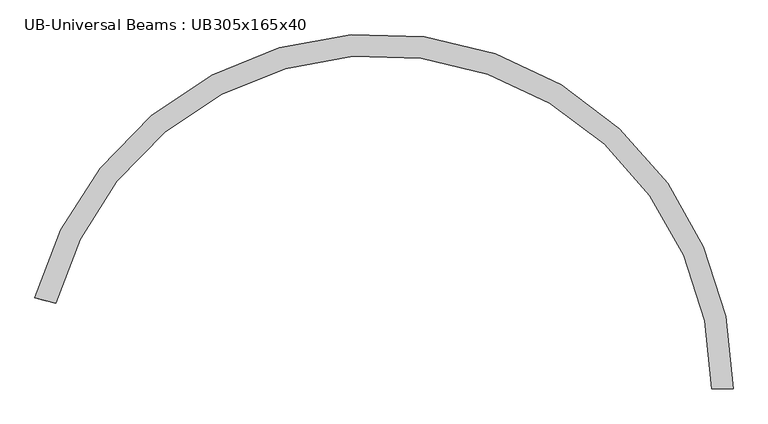
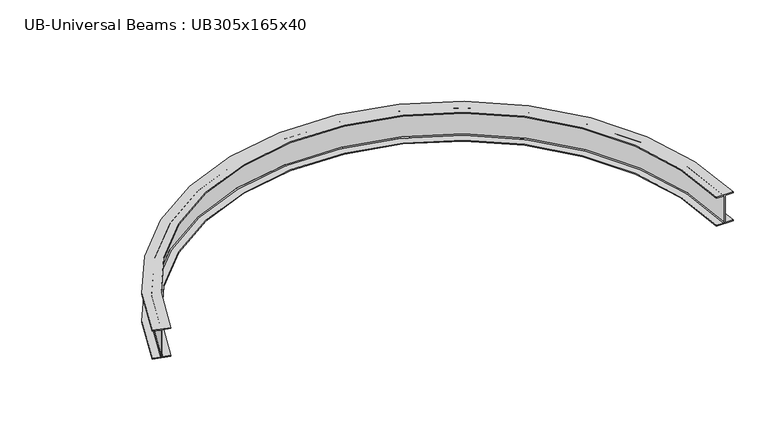
"""IFC4 building model written with IfcOpenShell, lengths in millimetres: beam geometry, UB-Universal Beams : UB305x165x40."""

from ifc_helpers import new_model, si_unit, point, frame, origin, place, context, project, spatial, polyline, circle_curve, ellipse_curve, trimmed, source, transform, mapped, element, save
from ifc_brep_helpers import plane_surface, cylinder_surface, revolved_surface, advanced_brep


def ub_universal_beams_ub305x165x40_4e4f8f72(model_context):
    return source(origin(), model_context, "Body", "AdvancedBrep", [
        advanced_brep(
        [(2724.4689627, -2641.9689627, -141.5), (2653.8689627, -2641.9689627, -141.5), (2644.9689627, -2641.9689627, -132.6), (2644.9689627, -2641.9689627, 132.6), (2653.8689627, -2641.9689627, 141.5), (2724.4689627, -2641.9689627, 141.5), (2724.4689627, -2641.9689627, 151.7), (2559.4689627, -2641.9689627, 151.7), (2559.4689627, -2641.9689627, 141.5), (2630.0689627, -2641.9689627, 141.5), (2638.9689627, -2641.9689627, 132.6), (2638.9689627, -2641.9689627, -132.6), (2630.0689627, -2641.9689627, -141.5), (2559.4689627, -2641.9689627, -141.5), (2559.4689627, -2641.9689627, -151.7), (2724.4689627, -2641.9689627, -151.7), (-2633.0924312, -1942.2866222, -141.5), (-2633.0924312, -1942.2866222, -151.7), (-2473.6264005, -1984.6609666, -151.7), (-2473.6264005, -1984.6609666, -141.5), (-2541.8585324, -1966.5298835, -141.5), (-2550.4600335, -1964.244237, -132.6), (-2550.4600335, -1964.244237, 132.6), (-2541.8585324, -1966.5298835, 141.5), (-2473.6264005, -1984.6609666, 141.5), (-2473.6264005, -1984.6609666, 151.7), (-2633.0924312, -1942.2866222, 151.7), (-2633.0924312, -1942.2866222, 141.5), (-2564.8602993, -1960.4177053, 141.5), (-2556.2587982, -1962.7033518, 132.6), (-2556.2587982, -1962.7033518, -132.6), (-2564.8602993, -1960.4177053, -141.5)],
        [
            (0, 1),
            (1, 2, circle_curve(frame((2653.8689627, -2641.9689627, -132.6), z_axis=(0.0, 1.0, 0.0), x_axis=(-1.0, 0.0, 0.0)), 8.9)),
            (2, 3),
            (3, 4, circle_curve(frame((2653.8689627, -2641.9689627, 132.6), z_axis=(0.0, 1.0, 0.0), x_axis=(-1.0, 0.0, 0.0)), 8.9)),
            (4, 5),
            (5, 6),
            (6, 7),
            (7, 8),
            (8, 9),
            (9, 10, circle_curve(frame((2630.0689627, -2641.9689627, 132.6), z_axis=(0.0, 1.0, 0.0), x_axis=(-1.0, 0.0, 0.0)), 8.9)),
            (10, 11),
            (11, 12, circle_curve(frame((2630.0689627, -2641.9689627, -132.6), z_axis=(0.0, 1.0, 0.0), x_axis=(-1.0, 0.0, 0.0)), 8.9)),
            (12, 13),
            (13, 14),
            (14, 15),
            (15, 0),
            (16, 17),
            (17, 18),
            (18, 19),
            (19, 20),
            (20, 21, circle_curve(frame((-2541.8585324, -1966.5298835, -132.6), z_axis=(0.2568142086103926, 0.9664607918875021, 0.0), x_axis=(0.9664607918875021, -0.2568142086103926, 0.0)), 8.9)),
            (21, 22),
            (22, 23, circle_curve(frame((-2541.8585324, -1966.5298835, 132.6), z_axis=(0.2568142086103926, 0.9664607918875021, 0.0), x_axis=(0.9664607918875021, -0.2568142086103926, 0.0)), 8.9)),
            (23, 24),
            (24, 25),
            (25, 26),
            (26, 27),
            (27, 28),
            (28, 29, circle_curve(frame((-2564.8602993, -1960.4177053, 132.6), z_axis=(0.2568142086103926, 0.9664607918875021, 0.0), x_axis=(0.9664607918875021, -0.2568142086103926, 0.0)), 8.9)),
            (29, 30),
            (30, 31, circle_curve(frame((-2564.8602993, -1960.4177053, -132.6), z_axis=(0.2568142086103926, 0.9664607918875021, 0.0), x_axis=(0.9664607918875021, -0.2568142086103926, 0.0)), 8.9)),
            (31, 16),
            (0, 16, circle_curve(frame((0.0, -2641.9689627, -141.5), z_axis=(0.0, 0.0, 1.0), x_axis=(0.0, 1.0, 0.0)), 2724.4689627)),
            (31, 1, circle_curve(frame((0.0, -2641.9689627, -141.5), z_axis=(0.0, 0.0, -1.0), x_axis=(0.0, 1.0, 0.0)), 2653.8689627)),
            (30, 2, circle_curve(frame((0.0, -2641.9689627, -132.6), z_axis=(0.0, 0.0, -1.0), x_axis=(0.0, 1.0, 0.0)), 2644.9689627)),
            (29, 3, circle_curve(frame((0.0, -2641.9689627, 132.6), z_axis=(0.0, 0.0, -1.0), x_axis=(0.0, 1.0, 0.0)), 2644.9689627)),
            (28, 4, circle_curve(frame((0.0, -2641.9689627, 141.5), z_axis=(0.0, 0.0, -1.0), x_axis=(0.0, 1.0, 0.0)), 2653.8689627)),
            (27, 5, circle_curve(frame((0.0, -2641.9689627, 141.5), z_axis=(0.0, 0.0, -1.0), x_axis=(0.0, 1.0, 0.0)), 2724.4689627)),
            (26, 6, circle_curve(frame((0.0, -2641.9689627, 151.7), z_axis=(0.0, 0.0, -1.0), x_axis=(0.0, 1.0, 0.0)), 2724.4689627)),
            (25, 7, circle_curve(frame((0.0, -2641.9689627, 151.7), z_axis=(0.0, 0.0, -1.0), x_axis=(0.0, 1.0, 0.0)), 2559.4689627)),
            (24, 8, circle_curve(frame((0.0, -2641.9689627, 141.5), z_axis=(0.0, 0.0, -1.0), x_axis=(0.0, 1.0, 0.0)), 2559.4689627)),
            (23, 9, circle_curve(frame((0.0, -2641.9689627, 141.5), z_axis=(0.0, 0.0, -1.0), x_axis=(0.0, 1.0, 0.0)), 2630.0689627)),
            (22, 10, circle_curve(frame((0.0, -2641.9689627, 132.6), z_axis=(0.0, 0.0, -1.0), x_axis=(0.0, 1.0, 0.0)), 2638.9689627)),
            (21, 11, circle_curve(frame((0.0, -2641.9689627, -132.6), z_axis=(0.0, 0.0, -1.0), x_axis=(0.0, 1.0, 0.0)), 2638.9689627)),
            (20, 12, circle_curve(frame((0.0, -2641.9689627, -141.5), z_axis=(0.0, 0.0, -1.0), x_axis=(0.0, 1.0, 0.0)), 2630.0689627)),
            (19, 13, circle_curve(frame((0.0, -2641.9689627, -141.5), z_axis=(0.0, 0.0, -1.0), x_axis=(0.0, 1.0, 0.0)), 2559.4689627)),
            (18, 14, circle_curve(frame((0.0, -2641.9689627, -151.7), z_axis=(0.0, 0.0, -1.0), x_axis=(0.0, 1.0, 0.0)), 2559.4689627)),
            (17, 15, circle_curve(frame((0.0, -2641.9689627, -151.7), z_axis=(0.0, 0.0, -1.0), x_axis=(0.0, 1.0, 0.0)), 2724.4689627)),
        ],
        [
            plane_surface(frame((2641.9689627, -2641.9689627, 0.0), z_axis=(0.0, -1.0, 0.0), x_axis=(0.0, 0.0, 1.0))),
            plane_surface(frame((-2553.3594159, -1963.4737944, 0.0), z_axis=(-0.25681420861039306, -0.9664607918875021, 0.0), x_axis=(0.0, 0.0, 1.0))),
            plane_surface(frame((0.0, -2641.9689627, -141.5), z_axis=(0.0, 0.0, 1.0), x_axis=(0.0, 1.0, 0.0))),
            revolved_surface(trimmed(ellipse_curve(frame((0.0, 11.9, -132.6), z_axis=(1.0, 0.0, 0.0), x_axis=(0.0, -1.0, 0.0)), 8.9, 8.9), [point((0.0, 3.0, -132.6))], [point((0.0, 11.9, -141.5))], True, "CARTESIAN"), (0.0, -2641.9689627, 0.0), (0.0, 0.0, -1.0)),
            cylinder_surface(frame((0.0, -2641.9689627, 0.0), z_axis=(0.0, 0.0, -1.0), x_axis=(0.0, 1.0, 0.0)), 2644.9689627),
            revolved_surface(trimmed(ellipse_curve(frame((0.0, 11.9, 132.6), z_axis=(1.0, 0.0, 0.0), x_axis=(0.0, -1.0, 0.0)), 8.9, 8.9), [point((0.0, 11.9, 141.5))], [point((0.0, 3.0, 132.6))], True, "CARTESIAN"), (0.0, -2641.9689627, 0.0), (0.0, 0.0, -1.0)),
            plane_surface(frame((0.0, -2641.9689627, 141.5), z_axis=(0.0, 0.0, -1.0), x_axis=(0.0, 1.0, 0.0))),
            cylinder_surface(frame((0.0, -2641.9689627, 0.0), z_axis=(0.0, 0.0, -1.0), x_axis=(0.0, 1.0, 0.0)), 2724.4689627),
            plane_surface(frame((0.0, -2641.9689627, 151.7), z_axis=(0.0, 0.0, 1.0), x_axis=(0.0, 1.0, 0.0))),
            revolved_surface(polyline([(0.0, -82.5, 141.5), (0.0, -82.5, 151.7)]), (0.0, -2641.9689627, 0.0), (0.0, 0.0, -1.0)),
            revolved_surface(trimmed(ellipse_curve(frame((0.0, -11.9, 132.6), z_axis=(1.0, 0.0, 0.0), x_axis=(0.0, -1.0, 0.0)), 8.9, 8.9), [point((0.0, -3.0, 132.6))], [point((0.0, -11.9, 141.5))], True, "CARTESIAN"), (0.0, -2641.9689627, 0.0), (0.0, 0.0, -1.0)),
            revolved_surface(polyline([(0.0, -3.0, -132.6), (0.0, -3.0, 132.6)]), (0.0, -2641.9689627, 0.0), (0.0, 0.0, -1.0)),
            revolved_surface(trimmed(ellipse_curve(frame((0.0, -11.9, -132.6), z_axis=(1.0, 0.0, 0.0), x_axis=(0.0, -1.0, 0.0)), 8.9, 8.9), [point((0.0, -11.9, -141.5))], [point((0.0, -3.0, -132.6))], True, "CARTESIAN"), (0.0, -2641.9689627, 0.0), (0.0, 0.0, -1.0)),
            revolved_surface(polyline([(0.0, -82.5, -151.7), (0.0, -82.5, -141.5)]), (0.0, -2641.9689627, 0.0), (0.0, 0.0, -1.0)),
            plane_surface(frame((0.0, -2641.9689627, -151.7), z_axis=(0.0, 0.0, -1.0), x_axis=(0.0, 1.0, 0.0))),
        ],
        [
            (0, [[1, 2, 3, 4, 5, 6, 7, 8, 9, 10, 11, 12, 13, 14, 15, 16]]),
            (1, [[17, 18, 19, 20, 21, 22, 23, 24, 25, 26, 27, 28, 29, 30, 31, 32]]),
            (2, [[-1, 33, -32, 34]]),
            (3, [[-2, -34, -31, 35]]),
            (4, [[-3, -35, -30, 36]]),
            (5, [[-4, -36, -29, 37]]),
            (6, [[-5, -37, -28, 38]]),
            (7, [[-6, -38, -27, 39]]),
            (8, [[-7, -39, -26, 40]]),
            (9, [[-8, -40, -25, 41]]),
            (6, [[-9, -41, -24, 42]]),
            (10, [[-10, -42, -23, 43]]),
            (11, [[-11, -43, -22, 44]]),
            (12, [[-12, -44, -21, 45]]),
            (2, [[-13, -45, -20, 46]]),
            (13, [[-14, -46, -19, 47]]),
            (14, [[-15, -47, -18, 48]]),
            (7, [[-16, -48, -17, -33]]),
        ],
    ),
    ])


if __name__ == "__main__":
    model = new_model("IFC4")
    model_context = context("Model", 3, world=origin())
    ifc_project = project(units=[si_unit("LENGTHUNIT", "METRE", prefix="MILLI")], contexts=[model_context])
    site = spatial("IfcSite", under=ifc_project)
    building = spatial("IfcBuilding", under=site)
    placement = place(None, origin())
    ub_universal_beams_ub305x165x40_shape = ub_universal_beams_ub305x165x40_4e4f8f72(model_context)
    element("IfcBeam", 1, ObjectType="UB-Universal Beams : UB305x165x40", at=placement, inside=building, context=model_context, shape_type="MappedRepresentation", body=[
        mapped(ub_universal_beams_ub305x165x40_shape, transform((0.0, 0.0, 0.0), x_axis=(1.0, 0.0, 0.0), y_axis=(0.0, 1.0, 0.0), z_axis=(0.0, 0.0, 1.0))),
    ])
    save(model, "model.ifc")

# Revit data of these elements
# Type "UB-Universal Beams : UB305x165x40"
#   Section Name Key = "UB305X165X40"
#   Width = 16.5 cm
#   Web Thickness = 0.6 cm
#   Web Fillet = 0.89 cm
#   Warping Constant = 164000.0 cm⁶
#   Torsional Moment of Inertia = 14.70 cm⁴
#   Section Area = 51.3 cm²
#   Plastic Modulus weak axis = 142.0 cm³
#   Plastic Modulus strong axis = 623.0 cm³
#   Nominal Weight = 40.2999 kgf/m
#   Moment of Inertia weak axis = 764.00 cm⁴
#   Moment of Inertia strong axis = 8503.00 cm⁴
#   Height = 30.34 cm
#   Flange Thickness = 1.02 cm
#   Elastic Modulus weak axis = 92.6 cm³
#   Elastic Modulus strong axis = 560.0 cm³
#   Centroid Vertical = 15.17 cm
#   Centroid Horizontal = 8.25 cm
#   Bolt Spacing = 9.0 cm
#   Length [instance default] = 1500 mm
#   Structural Material [instance default] = Metal - Steel 43-275
#   Type Comments = ""
#   Assembly Code = ""
# Element 1 (IfcBeam, "UB-Universal Beams : UB305x165x40")
#   Materials on its faces: "Metal - Steel 43-275"
# Materials
#   "Metal - Steel 43-275": class "Metal", colour RGB 247 247 247, transparency 0, Cost = 0
